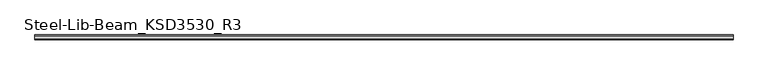
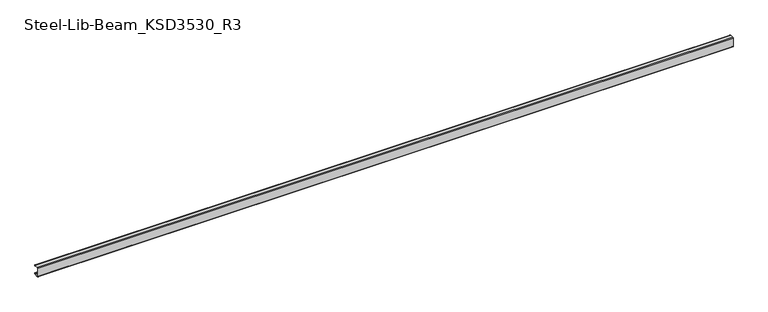
"""IFC4 building model written with IfcOpenShell, lengths in millimetres: beam geometry, Steel-Lib-Beam_KSD3530_R3 : BMS291_C-150×75x20x4.5."""

from ifc_helpers import new_model, si_unit, point, frame, frame_2d, origin, place, context, project, spatial, polyline, circle_curve, trimmed, segment, composite_curve, outline, extrude, source, transform, mapped, element, save


def steel_lib_beam_ksd3530_r3_8518c622(model_context):
    return source(origin(), model_context, "Body", "SweptSolid", [
        extrude(outline(composite_curve([segment(polyline([(50.0, 66.0), (50.0, 55.0), (45.5, 55.0), (45.5, 66.0)]), True, "CONTINUOUS"), segment(trimmed(circle_curve(frame_2d((41.0, 66.0)), 4.5), [point((45.5, 66.0))], [point((41.0, 70.5))], True, "CARTESIAN"), True, "CONTINUOUS"), segment(polyline([(41.0, 70.5), (-16.0, 70.5)]), True, "CONTINUOUS"), segment(trimmed(circle_curve(frame_2d((-16.0, 66.0)), 4.5), [point((-16.0, 70.5))], [point((-20.5, 66.0))], True, "CARTESIAN"), True, "CONTINUOUS"), segment(polyline([(-20.5, 66.0), (-20.5, -66.0)]), True, "CONTINUOUS"), segment(trimmed(circle_curve(frame_2d((-16.0, -66.0)), 4.5), [point((-20.5, -66.0))], [point((-16.0, -70.5))], True, "CARTESIAN"), True, "CONTINUOUS"), segment(polyline([(-16.0, -70.5), (41.0, -70.5)]), True, "CONTINUOUS"), segment(trimmed(circle_curve(frame_2d((41.0, -66.0)), 4.5), [point((41.0, -70.5))], [point((45.5, -66.0))], True, "CARTESIAN"), True, "CONTINUOUS"), segment(polyline([(45.5, -66.0), (45.5, -55.0), (50.0, -55.0), (50.0, -66.0)]), True, "CONTINUOUS"), segment(trimmed(circle_curve(frame_2d((41.0, -66.0)), 9.0), [point((50.0, -66.0))], [point((41.0, -75.0))], False, "CARTESIAN"), True, "CONTINUOUS"), segment(polyline([(41.0, -75.0), (-16.0, -75.0)]), True, "CONTINUOUS"), segment(trimmed(circle_curve(frame_2d((-16.0, -66.0)), 9.0), [point((-16.0, -75.0))], [point((-25.0, -66.0))], False, "CARTESIAN"), True, "CONTINUOUS"), segment(polyline([(-25.0, -66.0), (-25.0, 66.0)]), True, "CONTINUOUS"), segment(trimmed(circle_curve(frame_2d((-16.0, 66.0)), 9.0), [point((-25.0, 66.0))], [point((-16.0, 75.0))], False, "CARTESIAN"), True, "CONTINUOUS"), segment(polyline([(-16.0, 75.0), (41.0, 75.0)]), True, "CONTINUOUS"), segment(trimmed(circle_curve(frame_2d((41.0, 66.0)), 9.0), [point((41.0, 75.0))], [point((50.0, 66.0))], False, "CARTESIAN"), True, "CONTINUOUS")], self_intersect=False)), frame((-5215.0, 0.0, 0.0), z_axis=(1.0, 0.0, 0.0), x_axis=(0.0, 1.0, 0.0)), (0.0, 0.0, 1.0), 10430.0),
    ])


if __name__ == "__main__":
    model = new_model("IFC4")
    model_context = context("Model", 3, world=origin())
    ifc_project = project(units=[si_unit("LENGTHUNIT", "METRE", prefix="MILLI")], contexts=[model_context])
    site = spatial("IfcSite", under=ifc_project)
    building = spatial("IfcBuilding", under=site)
    placement = place(None, origin())
    steel_lib_beam_ksd3530_r3_shape = steel_lib_beam_ksd3530_r3_8518c622(model_context)
    element("IfcBeam", 1, ObjectType="Steel-Lib-Beam_KSD3530_R3 : BMS291_C-150×75x20x4.5", at=placement, inside=building, context=model_context, shape_type="MappedRepresentation", body=[
        mapped(steel_lib_beam_ksd3530_r3_shape, transform((0.0, 0.0, 0.0), x_axis=(1.0, 0.0, 0.0), y_axis=(0.0, 1.0, 0.0), z_axis=(0.0, 0.0, 1.0))),
    ])
    save(model, "model.ifc")

# Revit data of these elements
# Type "Steel-Lib-Beam_KSD3530_R3 : BMS291_C-150×75x20x4.5"
#   Keynote = "C-150×75x20x4.5"
#   SteelWeight = "Light"
#   x = 0.0250 m
#   t1 = 0.0090 m
#   t = 0.0045 m
#   Surface Area = 0.629834 m²/m
#   Section Area = 13.9688 cm²
#   Mass per Unit Length = 10.9655 kg/m
#   C = 0.0200 m
#   A = 0.0750 m
#   Length [instance default] = 1.5000 m
#   H = 0.1500 m
#   hec_material4 [instance default] = none
#   hec_material3 [instance default] = none
#   hec_material2 [instance default] = none
#   hec_material1 [instance default] = none
#   Structural Material [instance default] = Metal - Steel - Light Gauge
#   Assembly Code = ""
# Element 1 (IfcBeam, "Steel-Lib-Beam_KSD3530_R3 : BMS291_C-150×75x20x4.5")
#   Structural Material = none
# Materials
#   "Metal - Steel - Light Gauge": class "Metal", colour RGB 247 247 247, transparency 0
